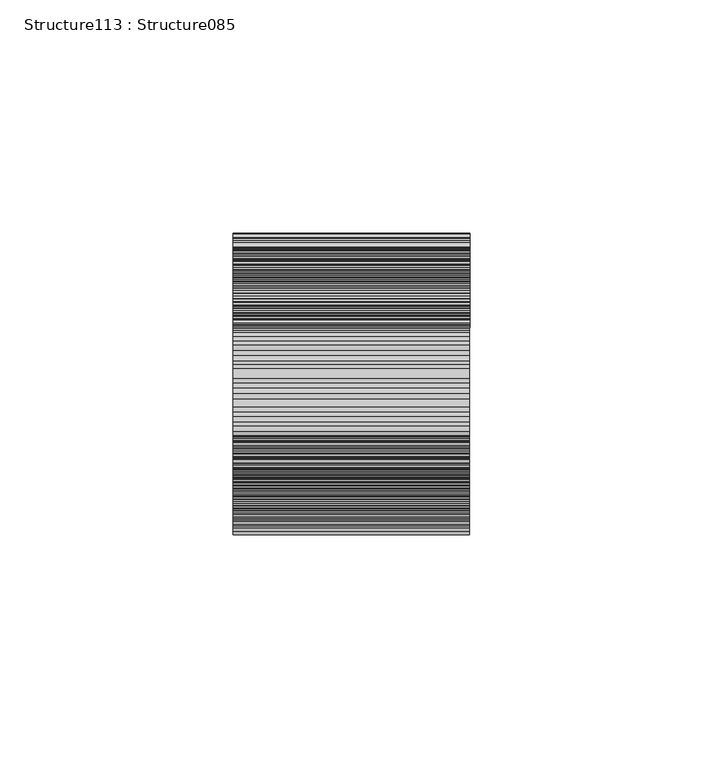
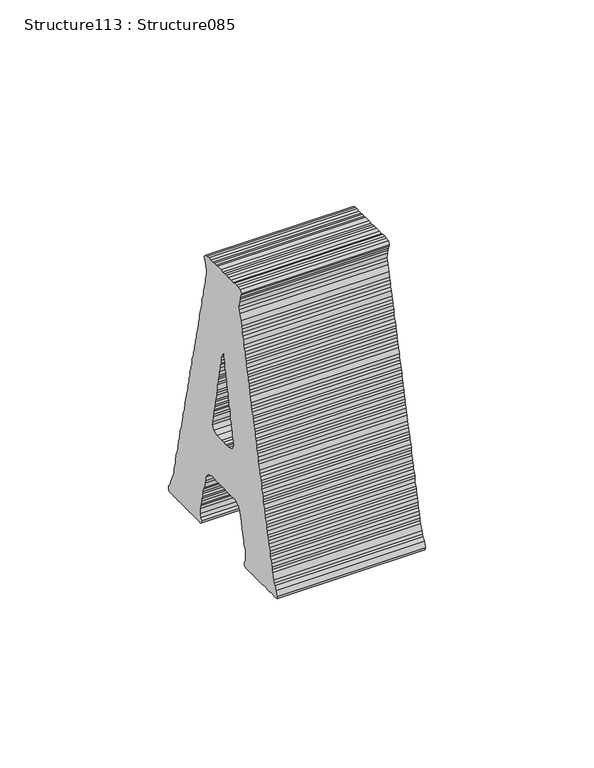
"""IFC4 building model written with IfcOpenShell, lengths in millimetres: proxy geometry, Structure113 : Structure085."""

import ifcopenshell
import ifcopenshell.guid

model = None  # the IFC model being written
_history = None  # IfcOwnerHistory: only IFC2X3 demands one
_inside = {}  # id of a spatial element -> (the spatial element, [elements in it])
_under = {}  # id of a project, library or spatial element -> (it, [spatial elements below it])
_declared = {}  # id of a project -> (the project, [libraries it declares])
_typed = {}  # id of a type object -> (the type object, [elements of that type])
_made_of = {}  # id of a material, layer set ... -> (it, [elements and type objects made of it])


def new_model(schema):
    """Start an empty IFC model of exactly this schema.

    Asked for "IFC4X3", IfcOpenShell would pick the latest addendum, in which some entities
    have other attributes; the version numbers below select the first issue.
    IFC2X3 requires an IfcOwnerHistory on every rooted entity: one is made here for all.
    """
    global model, _history
    if schema == "IFC4X3":
        model = ifcopenshell.file(schema_version=(4, 3, 0, 0))
    else:
        model = ifcopenshell.file(schema=schema)
    _inside.clear()
    _under.clear()
    _declared.clear()
    _typed.clear()
    _made_of.clear()
    _history = None
    if model.schema == "IFC2X3":
        org = make("IfcOrganization", Name="unknown")
        user = make(
            "IfcPersonAndOrganization",
            ThePerson=make("IfcPerson", FamilyName="unknown"),
            TheOrganization=org,
        )
        app = make(
            "IfcApplication",
            ApplicationDeveloper=org,
            Version="unknown",
            ApplicationFullName="unknown",
            ApplicationIdentifier="unknown",
        )
        _history = make(
            "IfcOwnerHistory",
            OwningUser=user,
            OwningApplication=app,
            ChangeAction="ADDED",
            CreationDate=0,
        )
    return model


def make(cls, **values):
    """One entity of the class cls with the attributes given. An attribute that is None is left unset."""
    return model.create_entity(
        cls, **{name: value for name, value in values.items() if value is not None}
    )


def rooted(cls, **values):
    """An entity with a GlobalId (a new one), such as an element, a storey or a relation."""
    return make(cls, GlobalId=ifcopenshell.guid.new(), OwnerHistory=_history, **values)


def si_unit(unit_type, name, prefix=None):
    """IfcSIUnit, for example si_unit("LENGTHUNIT", "METRE", prefix="MILLI")."""
    return make("IfcSIUnit", UnitType=unit_type, Prefix=prefix, Name=name)


def assignment(units):
    """IfcUnitAssignment: the units of a project."""
    return None if units is None else make("IfcUnitAssignment", Units=units)


def point(xyz):
    """IfcCartesianPoint."""
    return None if xyz is None else make("IfcCartesianPoint", Coordinates=xyz)


def direction(xyz):
    """IfcDirection."""
    return None if xyz is None else make("IfcDirection", DirectionRatios=xyz)


def frame(location, z_axis=None, x_axis=None):
    """IfcAxis2Placement3D, a coordinate frame: its origin and axes. An axis left out is left unset."""
    return make(
        "IfcAxis2Placement3D",
        Location=point(location),
        Axis=direction(z_axis),
        RefDirection=direction(x_axis),
    )


def origin():
    """The frame at (0, 0, 0) with its axes left unset."""
    return frame((0.0, 0.0, 0.0))


def place(relative_to, where):
    """IfcLocalPlacement: puts the frame where relative to a parent placement (None: the world)."""
    return make(
        "IfcLocalPlacement", PlacementRelTo=relative_to, RelativePlacement=where
    )


def context(
    kind, dimensions, precision=None, world=None, true_north=None, identifier=None
):
    """IfcGeometricRepresentationContext, for example the 3D "Model" context."""
    return make(
        "IfcGeometricRepresentationContext",
        ContextIdentifier=identifier,
        ContextType=kind,
        CoordinateSpaceDimension=dimensions,
        Precision=precision,
        WorldCoordinateSystem=world,
        TrueNorth=true_north,
    )


def project(units=None, contexts=None):
    """IfcProject with its units and contexts."""
    return rooted(
        "IfcProject",
        Name="project",
        RepresentationContexts=contexts,
        UnitsInContext=assignment(units),
    )


def spatial(cls, under=None, at=None, **own):
    """A site, building, storey or space (cls), placed at a placement, below another one or the project."""
    s = rooted(cls, ObjectPlacement=at, **own)
    if under is not None:
        _under.setdefault(under.id(), (under, []))[1].append(s)
    return s


def polyline(points):
    """IfcPolyline through the points."""
    return make("IfcPolyline", Points=[point(p) for p in points])


def outline(outer, holes=None, kind="AREA"):
    """IfcArbitraryClosedProfileDef: a profile drawn as a closed curve; with holes, ...WithVoids."""
    if holes is None:
        return make("IfcArbitraryClosedProfileDef", ProfileType=kind, OuterCurve=outer)
    return make(
        "IfcArbitraryProfileDefWithVoids",
        ProfileType=kind,
        OuterCurve=outer,
        InnerCurves=holes,
    )


def extrude(swept, where, along, depth):
    """IfcExtrudedAreaSolid: the profile swept, set in the frame where, extruded along a direction by depth."""
    return make(
        "IfcExtrudedAreaSolid",
        SweptArea=swept,
        Position=where,
        ExtrudedDirection=direction(along),
        Depth=depth,
    )


def shape(context_of_items, identifier, shape_type, items):
    """IfcShapeRepresentation: the items that make up one representation, for example the "Body"."""
    return make(
        "IfcShapeRepresentation",
        ContextOfItems=context_of_items,
        RepresentationIdentifier=identifier,
        RepresentationType=shape_type,
        Items=items,
    )


def source(mapping_origin, context_of_items, identifier, shape_type, items):
    """IfcRepresentationMap: a shape defined once, which mapped items show again and again."""
    return make(
        "IfcRepresentationMap",
        MappingOrigin=mapping_origin,
        MappedRepresentation=shape(context_of_items, identifier, shape_type, items),
    )


def transform(
    local_origin,
    x_axis=None,
    y_axis=None,
    z_axis=None,
    scale=None,
    scale2=None,
    scale3=None,
    uniform=True,
):
    """IfcCartesianTransformationOperator3D, or its non-uniform kind. x_axis, y_axis, z_axis: its Axis1, 2, 3."""
    if uniform:
        return make(
            "IfcCartesianTransformationOperator3D",
            Axis1=direction(x_axis),
            Axis2=direction(y_axis),
            LocalOrigin=point(local_origin),
            Scale=scale,
            Axis3=direction(z_axis),
        )
    return make(
        "IfcCartesianTransformationOperator3DnonUniform",
        Axis1=direction(x_axis),
        Axis2=direction(y_axis),
        LocalOrigin=point(local_origin),
        Scale=scale,
        Axis3=direction(z_axis),
        Scale2=scale2,
        Scale3=scale3,
    )


def mapped(mapping_source, mapping_target):
    """IfcMappedItem: shows the shape of a source again, moved by a transform."""
    return make(
        "IfcMappedItem", MappingSource=mapping_source, MappingTarget=mapping_target
    )


def made_of(thing, what):
    """Note that an element or type object is made of a material, layer set ...; save() writes the relation."""
    if what is not None:
        _made_of.setdefault(what.id(), (what, []))[1].append(thing)
    return thing


def element(
    cls,
    number,
    at=None,
    inside=None,
    cuts=None,
    type_object=None,
    material=None,
    context=None,
    identifier="Body",
    shape_type=None,
    held_by="IfcProductDefinitionShape",
    body=None,
    shapes=None,
    **own,
):
    """One element of the class cls, such as IfcWall. Its Tag is "e" and its number.

    at: its placement. inside: the storey or other place that contains it. cuts: it is an
    opening in that element (IfcRelVoidsElement). A single representation is given by context,
    identifier, shape_type and body (its items); several are given by shapes. held_by: the class
    of the entity that holds the representations. save() writes the other relations.
    """
    e = rooted(cls, Tag="e%d" % number, ObjectPlacement=at, **own)
    if body is not None:
        shapes = [shape(context, identifier, shape_type, body)]
    if shapes is not None:
        e.Representation = make(held_by, Representations=shapes)
    if inside is not None:
        _inside.setdefault(inside.id(), (inside, []))[1].append(e)
    if cuts is not None:
        rooted(
            "IfcRelVoidsElement", RelatingBuildingElement=cuts, RelatedOpeningElement=e
        )
    if type_object is not None:
        _typed.setdefault(type_object.id(), (type_object, []))[1].append(e)
    return made_of(e, material)


def aggregate(whole, parts):
    """IfcRelAggregates: a whole, such as a stair, and the parts it consists of."""
    return rooted("IfcRelAggregates", RelatingObject=whole, RelatedObjects=parts)


def save(model, path):
    """Write the relations noted so far, then the file.

    IfcRelAggregates (storeys below a building ...), IfcRelContainedInSpatialStructure (elements
    in a storey), IfcRelDefinesByType, IfcRelAssociatesMaterial and IfcRelDeclares: one each for
    every whole, place, type object, material and project.
    """
    for whole, parts in _under.values():
        aggregate(whole, parts)
    for where, things in _inside.values():
        rooted(
            "IfcRelContainedInSpatialStructure",
            RelatedElements=things,
            RelatingStructure=where,
        )
    for kind, things in _typed.values():
        rooted("IfcRelDefinesByType", RelatedObjects=things, RelatingType=kind)
    for what, things in _made_of.values():
        rooted("IfcRelAssociatesMaterial", RelatedObjects=things, RelatingMaterial=what)
    for by, libraries in _declared.values():
        rooted("IfcRelDeclares", RelatingContext=by, RelatedDefinitions=libraries)
    model.write(path)


def structure113_structure085_7526d104(model_context):
    return source(origin(), model_context, "Body", "SweptSolid", [
        extrude(outline(polyline([(0.9094651, 0.0), (2.0811665, -0.5237608), (2.9906316, -0.6522103), (4.1562841, -0.7856412), (5.1991801, -1.1709896), (5.9748585, -1.2994391), (7.1504738, -1.6901249), (8.1894559, -1.6901249), (9.3551083, -2.0804548), (10.2645735, -2.3423353), (11.4362748, -2.6042156), (12.3453841, -2.8611146), (13.3818755, -2.9895641), (14.1582655, -3.3802499), (15.4626861, -3.5086993), (16.3721513, -3.5086993), (17.5385154, -3.7705797), (19.491944, -4.4178086), (20.2718921, -4.679689), (21.3101626, -4.9369438), (22.3470097, -4.9369438), (23.2561191, -5.1988243), (24.4278204, -5.5891541), (25.4700048, -5.9745026), (26.6363689, -5.9745026), (27.4124031, -6.3648326), (28.7175354, -6.6270688), (30.535754, -7.0173987), (31.5743802, -7.1508296), (32.7400327, -7.4077286), (33.6555467, -7.7980584), (35.4741211, -7.7980584), (36.5102567, -7.5411595), (37.5492387, -7.2792791), (38.3288311, -6.8889491), (39.3671015, -6.3648326), (40.4099976, -7.2792791), (40.5395145, -8.1883884), (40.5395145, -9.0978535), (40.2826155, -10.269199), (40.2826155, -11.3067578), (40.5395145, -12.4781034), (40.4099976, -13.2541375), (40.5395145, -14.1682283), (40.5395145, -16.2437018), (40.2826155, -17.2816164), (40.2826155, -18.319531), (40.5395145, -19.4905207), (40.4099976, -20.6618662), (40.4099976, -22.3519911), (40.2826155, -23.5183552), (40.5395145, -24.4274645), (40.5395145, -25.5988101), (40.4099976, -26.5082752), (40.2826155, -27.6742835), (39.2382962, -28.4552991), (38.3288311, -27.9361639), (37.4197218, -27.6742835), (36.6397736, -27.5508154), (35.4741211, -27.2889351), (33.5199809, -26.8986051), (32.6112274, -27.1604855), (31.4448633, -27.4173845), (29.3636968, -28.1934188), (27.545834, -28.4552991), (26.5089869, -28.7171795), (25.3372855, -28.845629), (24.2943895, -29.1075095), (23.2561191, -29.6262888), (21.3101626, -29.7550941), (20.2718921, -30.0169745), (19.491944, -30.535754), (18.3202426, -30.535754), (17.2816164, -30.9211024), (16.3721513, -31.1829829), (15.3356599, -31.1829829), (14.1582655, -31.4452191), (13.1253323, -31.8355489), (12.2158672, -32.2258789), (11.4362748, -32.3543284), (10.2645735, -32.4877593), (9.3551083, -32.8731078), (8.1894559, -32.8731078), (7.1504738, -33.2637935), (6.2374505, -33.392243), (5.0714422, -33.6541234), (3.2475306, -34.3013523), (2.0811665, -34.3013523), (1.1720572, -34.5632327), (0.1334309, -34.8204876), (-1.0382704, -35.3442483), (-1.8178628, -35.4726978), (-2.8568449, -35.7345783), (-3.8990293, -35.8630278), (-5.0653934, -36.248732), (-5.8471206, -36.5106125), (-7.0166871, -36.5106125), (-8.1826954, -36.9009424), (-8.9644226, -37.0343733), (-10.1364798, -37.4247032), (-11.1690572, -37.5481713), (-12.2115974, -37.6766208), (-12.9915456, -37.938857), (-14.03373, -38.3291868), (-15.3292552, -38.4626178), (-16.3678815, -38.7195168), (-18.1861001, -39.1098467), (-19.3581573, -39.3667457), (-20.2672666, -39.7574314), (-21.4371888, -40.0193118), (-22.2189161, -40.2811923), (-23.1223323, -40.5430726), (-24.1648726, -40.5430726), (-25.465735, -41.0568706), (-26.5025822, -41.3191069), (-27.4173846, -41.4475563), (-28.4560108, -41.4475563), (-29.235959, -41.7094367), (-30.5311284, -42.0997667), (-31.3110766, -42.2282162), (-32.3536168, -42.6135646), (-33.5214042, -42.6135646), (-34.4308693, -43.1376813), (-35.3399786, -43.3995617), (-36.37647, -43.3995617), (-37.5424783, -43.6564606), (-38.7202285, -44.0467906), (-39.6236447, -44.3036896), (-40.405372, -44.5659258), (-41.5752942, -44.6943752), (-42.6139205, -45.0847052), (-43.7856218, -45.3465856), (-44.8221132, -45.3465856), (-45.7372714, -45.4800165), (-46.6406876, -45.9938145), (-47.812389, -46.2560507), (-48.8510152, -46.5179311), (-49.7601245, -46.5179311), (-50.6731478, -46.9082611), (-52.8777823, -47.5505085), (-53.7929405, -47.9461757), (-54.5689747, -48.3365055), (-55.738897, -49.1171654), (-57.5532016, -49.7647501), (-58.4665807, -49.5028697), (-58.5957419, -48.2030746), (-58.4665807, -47.4270404), (-58.3331498, -46.2560507), (-58.5957419, -45.2181361), (-58.5957419, -44.0467906), (-58.3331498, -43.0092318), (-58.3331498, -42.0997667), (-58.4665807, -41.0568706), (-58.4665807, -40.1477613), (-58.5957419, -38.8529477), (-58.5957419, -37.938857), (-58.4665807, -36.9009424), (-58.3331498, -35.7345783), (-58.5957419, -34.8204876), (-58.5957419, -31.8355489), (-58.3331498, -30.6642034), (-57.4297336, -30.1454241), (-56.6480063, -30.535754), (-55.6115149, -30.7976343), (-53.3972734, -30.7976343), (-52.3586471, -30.7976343), (-51.4495378, -30.535754), (-50.6731478, -30.1454241), (-49.3683714, -30.0169745), (-48.4592621, -29.7550941), (-47.5497969, -29.3644085), (-46.6406876, -29.1075095), (-45.6038405, -28.845629), (-43.2661308, -28.58873), (-41.5752942, -27.9361639), (-40.2762109, -27.6742835), (-38.9767716, -27.0270546), (-38.1950444, -26.1175895), (-37.4190102, -24.689345), (-37.6759092, -23.6517862), (-37.6759092, -21.5713313), (-37.5424783, -20.2715363), (-37.5424783, -17.5434968), (-37.6759092, -16.3721512), (-37.4190102, -15.4630419), (-37.5424783, -14.4201459), (-37.6759092, -13.382587), (-37.5424783, -12.4781034), (-37.4190102, -11.1733269), (-37.6759092, -10.3976485), (-38.0676623, -8.8359731), (-38.8476105, -8.0549575), (-40.2762109, -7.0173987), (-41.4422191, -7.0173987), (-42.6139205, -6.7604997), (-44.561656, -6.2363831), (-45.3472973, -5.7225851), (-46.5133056, -5.4607047), (-47.2932538, -5.3322552), (-48.33188, -5.3322552), (-49.3683714, -4.8081385), (-50.4126907, -4.679689), (-51.4495378, -4.5462581), (-52.3586471, -4.1609097), (-53.6595096, -3.7705797), (-55.3489229, -3.8990292), (-56.6480063, -4.2893592), (-57.2966585, -4.9369438), (-58.5957419, -4.1609097), (-58.4665807, -2.9895641), (-58.3331498, -1.9520053), (-58.3331498, 0.1288053), (-58.4665807, 1.1663641), (-58.4665807, 2.2092601), (-58.3331498, 3.113388), (-58.4665807, 4.0228532), (-58.4665807, 5.3276297), (-58.3331498, 6.1033081), (-58.4665807, 7.4031031), (-58.3331498, 8.1837629), (-58.5957419, 9.2216775), (-58.3331498, 10.393023), (-58.5957419, 11.5593872), (-58.4665807, 12.4684964), (-58.3331498, 13.5113925), (-58.3331498, 14.5489513), (-57.2966585, 14.939637), (-56.3875492, 14.6774008), (-55.738897, 14.0251904), (-54.5689747, 13.7732729), (-53.7929405, 13.3829429), (-52.6151903, 12.8588263), (-50.6731478, 11.9546985), (-49.8875066, 11.6928181), (-48.5941162, 11.5593872), (-47.5497969, 11.3021323), (-46.6406876, 11.0402519), (-45.8646534, 10.6549035), (-44.5616561, 10.5214725), (-42.6139205, 10.2645735), (-41.4422191, 9.8738878), (-40.5384471, 9.4835579), (-39.6236447, 9.2216775), (-38.4576364, 9.0882466), (-37.4190102, 8.9647785), (-36.5059869, 8.836329), (-35.6004358, 8.3125682), (-34.2956593, 8.1837629), (-33.3922431, 8.050332), (-32.3536168, 7.9218825), (-31.4405935, 7.5315525), (-30.4019673, 7.1462041), (-29.235959, 6.8843236), (-27.5447666, 6.6224432), (-26.3752002, 6.2317576), (-25.203143, 6.1033081), (-24.4235506, 5.8414276), (-23.3849244, 5.4560791), (-22.4793732, 5.3276297), (-21.3037579, 4.9369439), (-20.2672666, 4.9369439), (-19.3581573, 4.6750635), (-18.319531, 4.4131831), (-17.1474738, 4.1513026), (-15.2018732, 3.6375047), (-14.1632469, 3.3756243), (-13.1207067, 3.3756243), (-12.2115974, 2.9849386), (-11.3024881, 2.5946087), (-10.0012698, 2.5946087), (-9.2270147, 2.0808107), (-8.1826954, 2.0808107), (-7.0166871, 1.9473798), (-5.9745027, 1.4282446), (-5.0653934, 1.4282446), (-4.1619771, 0.9044837), (-2.8568449, 0.7760343), (-1.9473797, 0.7760343), (-0.7817273, 0.2572548), (0.0, 0.0), (0.9094651, 0.0)]), holes=[polyline([(-20.9137838, -13.9063479), (-20.9137838, -16.8912864), (-20.7903157, -18.0622762), (-21.0472147, -19.2336217), (-20.7903157, -20.1430868), (-20.9137838, -21.0472147), (-20.2672666, -22.99922), (-18.5817672, -23.6517862), (-17.2809048, -23.3899057), (-16.3678815, -23.1280253), (-15.4623303, -22.8657891), (-14.1632469, -22.99922), (-13.2480888, -22.4804406), (-12.2115974, -22.3519911), (-11.3024881, -22.2185602), (-10.393023, -21.8282304), (-9.3508386, -21.6997808), (-8.3122123, -21.6997808), (-7.146204, -21.5713313), (-6.3644768, -21.1806456), (-5.3276296, -20.9187652), (-4.2854452, -20.9187652), (-3.117302, -20.3999858), (-1.9473797, -20.3999858), (-1.0382704, -20.0096559), (-0.2561874, -19.8812064), (1.0389821, -19.7477754), (2.0811665, -19.4905207), (3.1180136, -19.2336217), (4.0274787, -19.1051722), (5.0714422, -19.1051722), (6.1082894, -18.5814114), (7.0177545, -18.4529619), (8.1894559, -18.4529619), (9.2216774, -18.0622762), (10.1368356, -17.8003957), (11.0463007, -17.8003957), (10.1368356, -17.1531669), (9.0928721, -16.7628369), (8.056025, -16.6343874), (6.8900167, -16.6343874), (6.1082894, -16.1102708), (4.9365881, -15.9818213), (3.1180136, -15.4630419), (1.8189302, -15.3345925), (0.9094651, -15.2061429), (0.0, -14.9442625), (-1.0382704, -14.8108316), (-2.2078369, -14.4201459), (-4.2854452, -14.2916963), (-5.3276296, -14.0347974), (-6.3644768, -13.9063479), (-8.1826954, -13.516018), (-9.2270147, -12.9919013), (-10.2638619, -12.9919013), (-11.1690572, -12.7350024), (-12.3446725, -12.6065529), (-13.1207067, -12.2162229), (-14.286715, -12.2162229), (-15.4623303, -11.8258931), (-17.2809048, -11.5640127), (-18.5817672, -11.3067578), (-20.1377496, -12.0877735), (-20.9137838, -13.9063479)])]), frame((-56111.7733116, 290724.5921101, -317.0048136), z_axis=(-0.9999998917542984, 0.00046528635450596156, 0.0), x_axis=(0.0, 0.0, 1.0)), (0.0, 0.0, 1.0), 50.8),
    ])


if __name__ == "__main__":
    model = new_model("IFC4")
    model_context = context("Model", 3, world=origin())
    ifc_project = project(units=[si_unit("LENGTHUNIT", "METRE", prefix="MILLI")], contexts=[model_context])
    site = spatial("IfcSite", under=ifc_project)
    building = spatial("IfcBuilding", under=site)
    placement = place(None, origin())
    structure113_structure085_shape = structure113_structure085_7526d104(model_context)
    element("IfcBuildingElementProxy", 1, Name="Structure113 : Structure085", ObjectType="Structure113 : Structure085", at=placement, inside=building, context=model_context, shape_type="MappedRepresentation", body=[
        mapped(structure113_structure085_shape, transform((0.0, 0.0, 0.0), x_axis=(1.0, 0.0, 0.0), y_axis=(0.0, 1.0, 0.0), z_axis=(0.0, 0.0, 1.0))),
    ])
    save(model, "model.ifc")

# Revit data of these elements
# Type "Structure113 : Structure085"
#   NameOverride = "Structure085"
# Element 1 (IfcBuildingElementProxy, "Structure113 : Structure085")
#   Materials on its faces: "BRUSHED ALUMINUM LETTERING"
# Materials
#   "BRUSHED ALUMINUM LETTERING": class "Unassigned", colour RGB 169 181 186, transparency 0, Cost = 0
